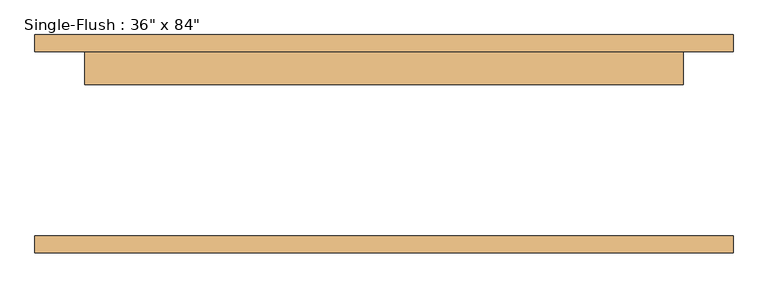
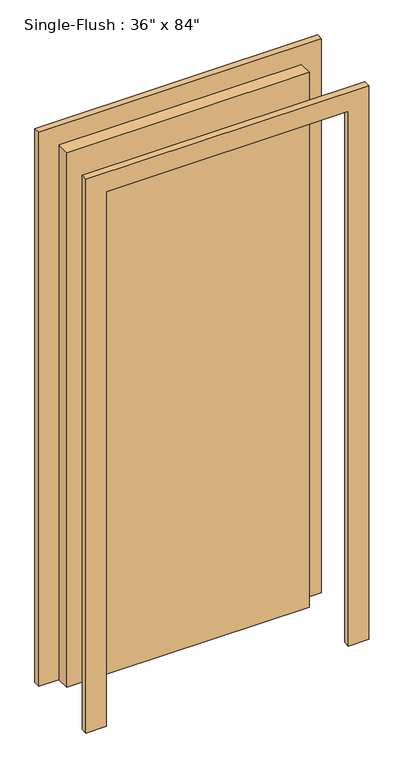
"""IFC4 building model written with IfcOpenShell, lengths in millimetres: door geometry."""

from ifc_helpers import new_model, si_unit, frame, origin, origin_with_axes, place, context, project, spatial, polyline, outline, extrude, source, transform, mapped, element, save


def door_23c500ab(model_context):
    return source(origin(), model_context, "Body", "SweptSolid", [
        extrude(outline(polyline([(2209.8, -533.4), (0.0, -533.4), (0.0, -457.2), (2133.6, -457.2), (2133.6, 457.2), (0.0, 457.2), (0.0, 533.4), (2209.8, 533.4), (2209.8, -533.4)])), frame((0.0, 141.2875, 0.0), z_axis=(0.0, 1.0, 0.0), x_axis=(0.0, 0.0, 1.0)), (0.0, 0.0, 1.0), 25.4),
        extrude(outline(polyline([(2209.8, 533.4), (2209.8, -533.4), (0.0, -533.4), (0.0, -457.2), (2133.6, -457.2), (2133.6, 457.2), (0.0, 457.2), (0.0, 533.4), (2209.8, 533.4)])), frame((0.0, -166.6875, 0.0), z_axis=(0.0, 1.0, 0.0), x_axis=(0.0, 0.0, 1.0)), (0.0, 0.0, 1.0), 25.4),
        extrude(outline(polyline([(457.2, 90.4875), (-457.2, 90.4875), (-457.2, 141.2875), (457.2, 141.2875), (457.2, 90.4875)])), origin_with_axes(), (0.0, 0.0, 1.0), 2133.6),
    ])


if __name__ == "__main__":
    model = new_model("IFC4")
    model_context = context("Model", 3, world=origin())
    ifc_project = project(units=[si_unit("LENGTHUNIT", "METRE", prefix="MILLI")], contexts=[model_context])
    site = spatial("IfcSite", under=ifc_project)
    building = spatial("IfcBuilding", under=site)
    placement = place(None, origin())
    door_shape = door_23c500ab(model_context)
    element("IfcDoor", 1, ObjectType="Single-Flush : 36\" x 84\"", at=placement, inside=building, context=model_context, shape_type="MappedRepresentation", body=[
        mapped(door_shape, transform((0.0, 0.0, 0.0), x_axis=(1.0, 0.0, 0.0), y_axis=(0.0, 1.0, 0.0), z_axis=(0.0, 0.0, 1.0))),
    ])
    save(model, "model.ifc")

# Revit data of these elements
# Type "Single-Flush : 36\" x 84\""
#   Type Mark = "1"
#   Assembly Code = "C1020"
#   Thickness = 0' - 2"
#   Height = 7' - 0"
#   Trim Projection Ext = 0' - 1"
#   Trim Projection Int = 0' - 1"
#   Trim Width = 0' - 3"
#   Width = 3' - 0"
#   Door Material = PAINTED STEEL C CHANNEL
#   Frame Material = PAINTED STEEL C CHANNEL
#   Function = (empty or 0)
#   Wall Closure = (empty or 0)
# Element 1 (IfcDoor, "Single-Flush : 36\" x 84\"")
#   Materials on its faces: "PAINTED STEEL C CHANNEL"
# Materials
#   "PAINTED STEEL C CHANNEL": class "Generic", colour RGB 88 62 61, transparency 0, Cost = 0
